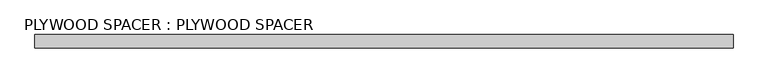
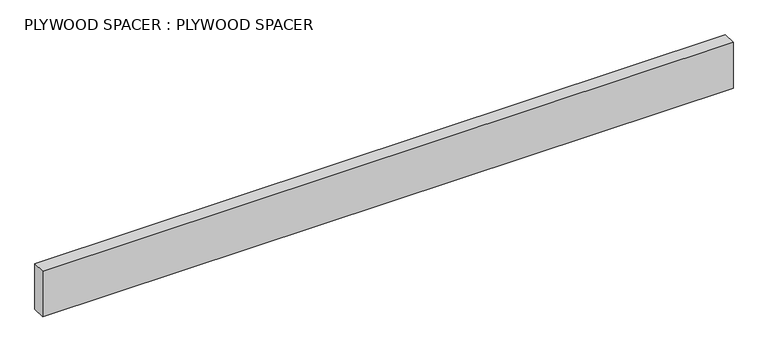
"""IFC4 building model written with IfcOpenShell, lengths in millimetres: proxy geometry, PLYWOOD SPACER : PLYWOOD SPACER."""

import ifcopenshell
import ifcopenshell.guid

model = None  # the IFC model being written
_history = None  # IfcOwnerHistory: only IFC2X3 demands one
_inside = {}  # id of a spatial element -> (the spatial element, [elements in it])
_under = {}  # id of a project, library or spatial element -> (it, [spatial elements below it])
_declared = {}  # id of a project -> (the project, [libraries it declares])
_typed = {}  # id of a type object -> (the type object, [elements of that type])
_made_of = {}  # id of a material, layer set ... -> (it, [elements and type objects made of it])


def new_model(schema):
    """Start an empty IFC model of exactly this schema.

    Asked for "IFC4X3", IfcOpenShell would pick the latest addendum, in which some entities
    have other attributes; the version numbers below select the first issue.
    IFC2X3 requires an IfcOwnerHistory on every rooted entity: one is made here for all.
    """
    global model, _history
    if schema == "IFC4X3":
        model = ifcopenshell.file(schema_version=(4, 3, 0, 0))
    else:
        model = ifcopenshell.file(schema=schema)
    _inside.clear()
    _under.clear()
    _declared.clear()
    _typed.clear()
    _made_of.clear()
    _history = None
    if model.schema == "IFC2X3":
        org = make("IfcOrganization", Name="unknown")
        user = make(
            "IfcPersonAndOrganization",
            ThePerson=make("IfcPerson", FamilyName="unknown"),
            TheOrganization=org,
        )
        app = make(
            "IfcApplication",
            ApplicationDeveloper=org,
            Version="unknown",
            ApplicationFullName="unknown",
            ApplicationIdentifier="unknown",
        )
        _history = make(
            "IfcOwnerHistory",
            OwningUser=user,
            OwningApplication=app,
            ChangeAction="ADDED",
            CreationDate=0,
        )
    return model


def make(cls, **values):
    """One entity of the class cls with the attributes given. An attribute that is None is left unset."""
    return model.create_entity(
        cls, **{name: value for name, value in values.items() if value is not None}
    )


def rooted(cls, **values):
    """An entity with a GlobalId (a new one), such as an element, a storey or a relation."""
    return make(cls, GlobalId=ifcopenshell.guid.new(), OwnerHistory=_history, **values)


def si_unit(unit_type, name, prefix=None):
    """IfcSIUnit, for example si_unit("LENGTHUNIT", "METRE", prefix="MILLI")."""
    return make("IfcSIUnit", UnitType=unit_type, Prefix=prefix, Name=name)


def assignment(units):
    """IfcUnitAssignment: the units of a project."""
    return None if units is None else make("IfcUnitAssignment", Units=units)


def point(xyz):
    """IfcCartesianPoint."""
    return None if xyz is None else make("IfcCartesianPoint", Coordinates=xyz)


def direction(xyz):
    """IfcDirection."""
    return None if xyz is None else make("IfcDirection", DirectionRatios=xyz)


def frame(location, z_axis=None, x_axis=None):
    """IfcAxis2Placement3D, a coordinate frame: its origin and axes. An axis left out is left unset."""
    return make(
        "IfcAxis2Placement3D",
        Location=point(location),
        Axis=direction(z_axis),
        RefDirection=direction(x_axis),
    )


def origin():
    """The frame at (0, 0, 0) with its axes left unset."""
    return frame((0.0, 0.0, 0.0))


def place(relative_to, where):
    """IfcLocalPlacement: puts the frame where relative to a parent placement (None: the world)."""
    return make(
        "IfcLocalPlacement", PlacementRelTo=relative_to, RelativePlacement=where
    )


def context(
    kind, dimensions, precision=None, world=None, true_north=None, identifier=None
):
    """IfcGeometricRepresentationContext, for example the 3D "Model" context."""
    return make(
        "IfcGeometricRepresentationContext",
        ContextIdentifier=identifier,
        ContextType=kind,
        CoordinateSpaceDimension=dimensions,
        Precision=precision,
        WorldCoordinateSystem=world,
        TrueNorth=true_north,
    )


def project(units=None, contexts=None):
    """IfcProject with its units and contexts."""
    return rooted(
        "IfcProject",
        Name="project",
        RepresentationContexts=contexts,
        UnitsInContext=assignment(units),
    )


def spatial(cls, under=None, at=None, **own):
    """A site, building, storey or space (cls), placed at a placement, below another one or the project."""
    s = rooted(cls, ObjectPlacement=at, **own)
    if under is not None:
        _under.setdefault(under.id(), (under, []))[1].append(s)
    return s


def polyline(points):
    """IfcPolyline through the points."""
    return make("IfcPolyline", Points=[point(p) for p in points])


def outline(outer, holes=None, kind="AREA"):
    """IfcArbitraryClosedProfileDef: a profile drawn as a closed curve; with holes, ...WithVoids."""
    if holes is None:
        return make("IfcArbitraryClosedProfileDef", ProfileType=kind, OuterCurve=outer)
    return make(
        "IfcArbitraryProfileDefWithVoids",
        ProfileType=kind,
        OuterCurve=outer,
        InnerCurves=holes,
    )


def extrude(swept, where, along, depth):
    """IfcExtrudedAreaSolid: the profile swept, set in the frame where, extruded along a direction by depth."""
    return make(
        "IfcExtrudedAreaSolid",
        SweptArea=swept,
        Position=where,
        ExtrudedDirection=direction(along),
        Depth=depth,
    )


def shape(context_of_items, identifier, shape_type, items):
    """IfcShapeRepresentation: the items that make up one representation, for example the "Body"."""
    return make(
        "IfcShapeRepresentation",
        ContextOfItems=context_of_items,
        RepresentationIdentifier=identifier,
        RepresentationType=shape_type,
        Items=items,
    )


def source(mapping_origin, context_of_items, identifier, shape_type, items):
    """IfcRepresentationMap: a shape defined once, which mapped items show again and again."""
    return make(
        "IfcRepresentationMap",
        MappingOrigin=mapping_origin,
        MappedRepresentation=shape(context_of_items, identifier, shape_type, items),
    )


def transform(
    local_origin,
    x_axis=None,
    y_axis=None,
    z_axis=None,
    scale=None,
    scale2=None,
    scale3=None,
    uniform=True,
):
    """IfcCartesianTransformationOperator3D, or its non-uniform kind. x_axis, y_axis, z_axis: its Axis1, 2, 3."""
    if uniform:
        return make(
            "IfcCartesianTransformationOperator3D",
            Axis1=direction(x_axis),
            Axis2=direction(y_axis),
            LocalOrigin=point(local_origin),
            Scale=scale,
            Axis3=direction(z_axis),
        )
    return make(
        "IfcCartesianTransformationOperator3DnonUniform",
        Axis1=direction(x_axis),
        Axis2=direction(y_axis),
        LocalOrigin=point(local_origin),
        Scale=scale,
        Axis3=direction(z_axis),
        Scale2=scale2,
        Scale3=scale3,
    )


def mapped(mapping_source, mapping_target):
    """IfcMappedItem: shows the shape of a source again, moved by a transform."""
    return make(
        "IfcMappedItem", MappingSource=mapping_source, MappingTarget=mapping_target
    )


def made_of(thing, what):
    """Note that an element or type object is made of a material, layer set ...; save() writes the relation."""
    if what is not None:
        _made_of.setdefault(what.id(), (what, []))[1].append(thing)
    return thing


def element(
    cls,
    number,
    at=None,
    inside=None,
    cuts=None,
    type_object=None,
    material=None,
    context=None,
    identifier="Body",
    shape_type=None,
    held_by="IfcProductDefinitionShape",
    body=None,
    shapes=None,
    **own,
):
    """One element of the class cls, such as IfcWall. Its Tag is "e" and its number.

    at: its placement. inside: the storey or other place that contains it. cuts: it is an
    opening in that element (IfcRelVoidsElement). A single representation is given by context,
    identifier, shape_type and body (its items); several are given by shapes. held_by: the class
    of the entity that holds the representations. save() writes the other relations.
    """
    e = rooted(cls, Tag="e%d" % number, ObjectPlacement=at, **own)
    if body is not None:
        shapes = [shape(context, identifier, shape_type, body)]
    if shapes is not None:
        e.Representation = make(held_by, Representations=shapes)
    if inside is not None:
        _inside.setdefault(inside.id(), (inside, []))[1].append(e)
    if cuts is not None:
        rooted(
            "IfcRelVoidsElement", RelatingBuildingElement=cuts, RelatedOpeningElement=e
        )
    if type_object is not None:
        _typed.setdefault(type_object.id(), (type_object, []))[1].append(e)
    return made_of(e, material)


def aggregate(whole, parts):
    """IfcRelAggregates: a whole, such as a stair, and the parts it consists of."""
    return rooted("IfcRelAggregates", RelatingObject=whole, RelatedObjects=parts)


def save(model, path):
    """Write the relations noted so far, then the file.

    IfcRelAggregates (storeys below a building ...), IfcRelContainedInSpatialStructure (elements
    in a storey), IfcRelDefinesByType, IfcRelAssociatesMaterial and IfcRelDeclares: one each for
    every whole, place, type object, material and project.
    """
    for whole, parts in _under.values():
        aggregate(whole, parts)
    for where, things in _inside.values():
        rooted(
            "IfcRelContainedInSpatialStructure",
            RelatedElements=things,
            RelatingStructure=where,
        )
    for kind, things in _typed.values():
        rooted("IfcRelDefinesByType", RelatedObjects=things, RelatingType=kind)
    for what, things in _made_of.values():
        rooted("IfcRelAssociatesMaterial", RelatedObjects=things, RelatingMaterial=what)
    for by, libraries in _declared.values():
        rooted("IfcRelDeclares", RelatingContext=by, RelatedDefinitions=libraries)
    model.write(path)


def plywood_spacer_plywood_spacer_aff279fe(model_context):
    return source(origin(), model_context, "Body", "SweptSolid", [
        extrude(outline(polyline([(12382.7678845, -4586.7425368), (12382.7678845, -4548.6425368), (14383.0178845, -4548.6425368), (14383.0178845, -4586.7425368), (12382.7678845, -4586.7425368)])), frame((0.0, 0.0, 39019.0959974), z_axis=(0.0, 0.0, 1.0), x_axis=(1.0, 0.0, 0.0)), (0.0, 0.0, 1.0), 139.7),
    ])


if __name__ == "__main__":
    model = new_model("IFC4")
    model_context = context("Model", 3, world=origin())
    ifc_project = project(units=[si_unit("LENGTHUNIT", "METRE", prefix="MILLI")], contexts=[model_context])
    site = spatial("IfcSite", under=ifc_project)
    building = spatial("IfcBuilding", under=site)
    placement = place(None, origin())
    plywood_spacer_plywood_spacer_shape = plywood_spacer_plywood_spacer_aff279fe(model_context)
    element("IfcBuildingElementProxy", 1, Name="PLYWOOD SPACER : PLYWOOD SPACER", ObjectType="PLYWOOD SPACER : PLYWOOD SPACER", at=placement, inside=building, context=model_context, shape_type="MappedRepresentation", body=[
        mapped(plywood_spacer_plywood_spacer_shape, transform((0.0, 0.0, 0.0), x_axis=(1.0, 0.0, 0.0), y_axis=(0.0, 1.0, 0.0), z_axis=(0.0, 0.0, 1.0))),
    ])
    save(model, "model.ifc")

# Revit data of these elements
# Type "PLYWOOD SPACER : PLYWOOD SPACER"
#   NameOverride = "PLYWOOD SPACER"
# Element 1 (IfcBuildingElementProxy, "PLYWOOD SPACER : PLYWOOD SPACER")
#   Materials on its faces: "WOOD BLOCKING AS REQUIRED"
# Materials
#   "WOOD BLOCKING AS REQUIRED": class "Unassigned", colour RGB 166 124 85, transparency 0, Cost = 0
